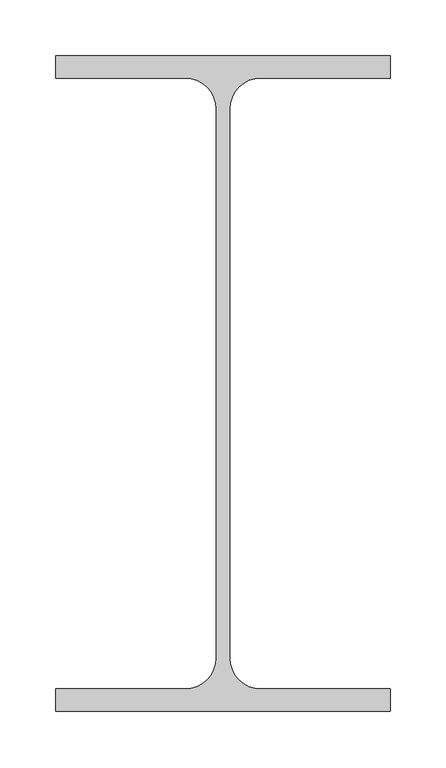
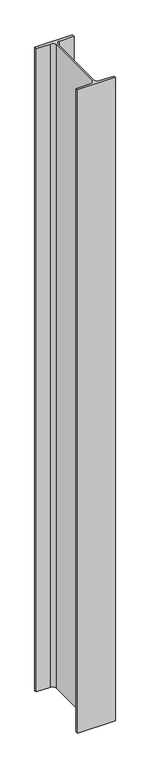
"""IFC4 building model written with IfcOpenShell, lengths in millimetres: column geometry, 0912_Steel Column_H_KSD3502 : H_SC_ASC_H-588x300x12x20."""

from ifc_helpers import new_model, si_unit, point, frame, frame_2d, origin, place, context, project, spatial, polyline, circle_curve, trimmed, segment, composite_curve, outline, extrude, source, transform, mapped, element, save


def column_190025ee(model_context):
    return source(origin(), model_context, "Body", "SweptSolid", [
        extrude(outline(composite_curve([segment(polyline([(150.0, 294.0), (150.0, 274.0), (34.0, 274.0)]), True, "CONTINUOUS"), segment(trimmed(circle_curve(frame_2d((34.0, 246.0)), 28.0), [point((34.0, 274.0))], [point((6.0, 246.0))], True, "CARTESIAN"), True, "CONTINUOUS"), segment(polyline([(6.0, 246.0), (6.0, -246.0)]), True, "CONTINUOUS"), segment(trimmed(circle_curve(frame_2d((34.0, -246.0)), 28.0), [point((6.0, -246.0))], [point((34.0, -274.0))], True, "CARTESIAN"), True, "CONTINUOUS"), segment(polyline([(34.0, -274.0), (150.0, -274.0), (150.0, -294.0), (-150.0, -294.0), (-150.0, -274.0), (-34.0, -274.0)]), True, "CONTINUOUS"), segment(trimmed(circle_curve(frame_2d((-34.0, -246.0)), 28.0), [point((-34.0, -274.0))], [point((-6.0, -246.0))], True, "CARTESIAN"), True, "CONTINUOUS"), segment(polyline([(-6.0, -246.0), (-6.0, 246.0)]), True, "CONTINUOUS"), segment(trimmed(circle_curve(frame_2d((-34.0, 246.0)), 28.0), [point((-6.0, 246.0))], [point((-34.0, 274.0))], True, "CARTESIAN"), True, "CONTINUOUS"), segment(polyline([(-34.0, 274.0), (-150.0, 274.0), (-150.0, 294.0), (150.0, 294.0)]), True, "CONTINUOUS")], self_intersect=False)), frame((0.0, 0.0, 11909.9720055), z_axis=(0.0, 0.0, 1.0), x_axis=(1.0, 0.0, 0.0)), (0.0, 0.0, 1.0), 5390.0),
    ])


if __name__ == "__main__":
    model = new_model("IFC4")
    model_context = context("Model", 3, world=origin())
    ifc_project = project(units=[si_unit("LENGTHUNIT", "METRE", prefix="MILLI")], contexts=[model_context])
    site = spatial("IfcSite", under=ifc_project)
    building = spatial("IfcBuilding", under=site)
    placement = place(None, origin())
    column_shape = column_190025ee(model_context)
    element("IfcColumn", 1, ObjectType="0912_Steel Column_H_KSD3502 : H_SC_ASC_H-588x300x12x20", at=placement, inside=building, context=model_context, shape_type="MappedRepresentation", body=[
        mapped(column_shape, transform((0.0, 0.0, 0.0), x_axis=(1.0, 0.0, 0.0), y_axis=(0.0, 1.0, 0.0), z_axis=(0.0, 0.0, 1.0))),
    ])
    save(model, "model.ifc")

# Revit data of these elements
# Type "0912_Steel Column_H_KSD3502 : H_SC_ASC_H-588x300x12x20"
#   H_WM Code_1 = "S01AA002-00001 | Main Steel Structure Fabrication Work | Shelter/Building | Medium Steel - Standard (90KG/M>Weight≥30KG/M) | Material: (   )"
#   H_WM Code_2 = "S03AA028-00001 | Main Steel Structure Erection Work | Shelter/Building | Medium Steel (90KG/M>Weight≥30KG/M) | Material: (   )"
#   H_WM Code_3 = "S01AA010-00001 | Main Steel Structure Fabrication Work | Shelter/Building | Steel Painting/Coating | for Non-Fireproofed Steel Surface, Surface Preparation, Primer, Second & Final Coat | Material: (   )"
#   H_Q'ty Cal Type Tag = "SC-Q2"
#   Width = 30.0 cm
#   Web Thickness = 1.2 cm
#   Web Fillet = 2.8 cm
#   Warping Constant = 7259040.0 cm⁶
#   Torsional Moment of Inertia = 192.717 cm⁴
#   Section Area = 192.5 cm²
#   Plastic Modulus weak axis = 928.0 cm³
#   Plastic Modulus strong axis = 4490.0 cm³
#   Perimeter = 2.30 m²/m
#   Nominal Weight = 151.00 kgf/m
#   Moment of Inertia weak axis = 9020.00 cm⁴
#   Moment of Inertia strong axis = 118000.00 cm⁴
#   Height = 58.8 cm
#   Flange Thickness = 2.0 cm
#   Elastic Modulus weak axis = 601.0 cm³
#   Elastic Modulus strong axis = 4020.0 cm³
#   Centroid Vertical = 29.4 cm
#   Centroid Horizontal = 15.0 cm
#   Structural Material [instance default] = Steel, 45-345
#   Section Name Key = ""
#   Bolt Spacing = 0
#   Assembly Code = ""
# Element 1 (IfcColumn, "0912_Steel Column_H_KSD3502 : H_SC_ASC_H-588x300x12x20")
#   Structural Material = none
# Materials
#   "Steel, 45-345": class "Metal", colour RGB 189 187 185, transparency 0, Description = "Steel 345 MPa", Cost = 0
